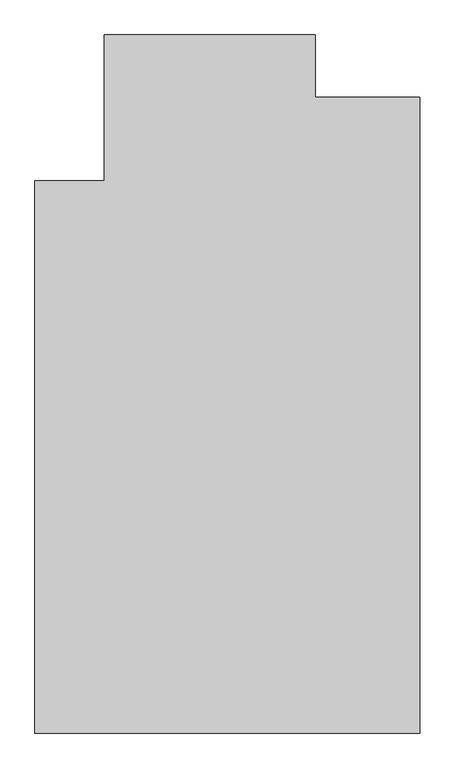
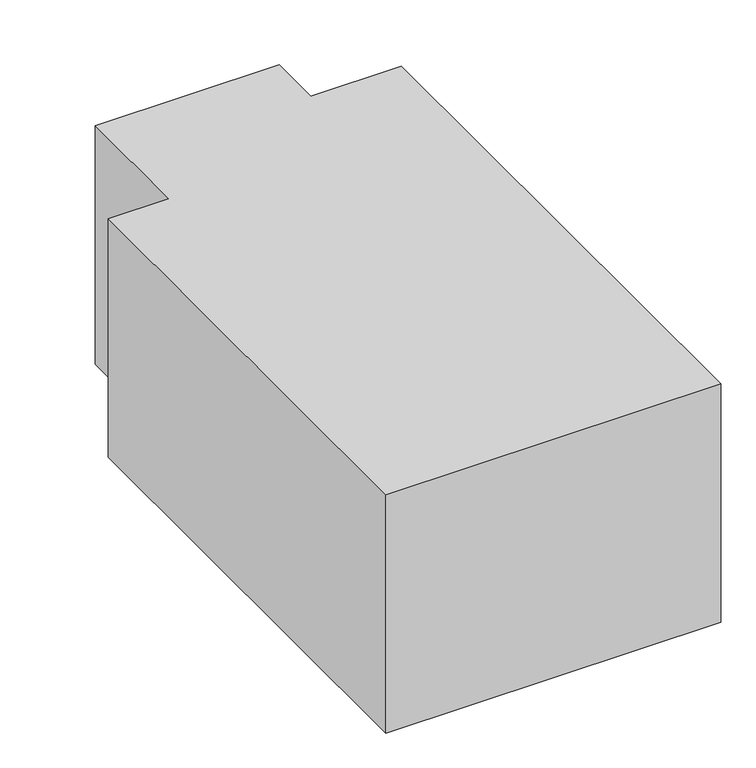
"""IFC4 building model written with IfcOpenShell, lengths in millimetres: proxy geometry, 0_3d."""

from ifc_helpers import new_model, si_unit, origin, origin_with_axes, place, context, project, spatial, polyline, outline, extrude, source, transform, mapped, element, save


def generic_models_0f8ef8ea(model_context):
    return source(origin(), model_context, "Body", "SweptSolid", [
        extrude(outline(polyline([(3320.0, 0.0), (0.0, 0.0), (0.0, 4765.0), (600.0, 4765.0), (600.0, 6025.0), (2420.0, 6025.0), (2420.0, 5485.0), (3320.0, 5485.0), (3320.0, 0.0)])), origin_with_axes(), (0.0, 0.0, 1.0), 2500.0),
    ])


if __name__ == "__main__":
    model = new_model("IFC4")
    model_context = context("Model", 3, world=origin())
    ifc_project = project(units=[si_unit("LENGTHUNIT", "METRE", prefix="MILLI")], contexts=[model_context])
    site = spatial("IfcSite", under=ifc_project)
    building = spatial("IfcBuilding", under=site)
    placement = place(None, origin())
    generic_models_shape = generic_models_0f8ef8ea(model_context)
    element("IfcBuildingElementProxy", 1, Name="0_3d", ObjectType="0_3d", at=placement, inside=building, context=model_context, shape_type="MappedRepresentation", body=[
        mapped(generic_models_shape, transform((0.0, 0.0, 0.0), x_axis=(1.0, 0.0, 0.0), y_axis=(0.0, 1.0, 0.0), z_axis=(0.0, 0.0, 1.0))),
    ])
    save(model, "model.ifc")

# Revit data of these elements
# Element 1 (IfcBuildingElementProxy, "0_3d")
#   Materials on its faces: "*1"
# Materials
#   "*1": class "Unassigned", colour RGB 175 175 175, transparency 0
